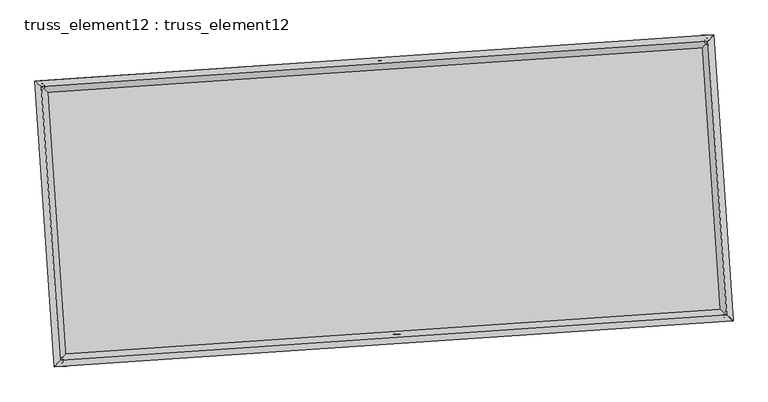
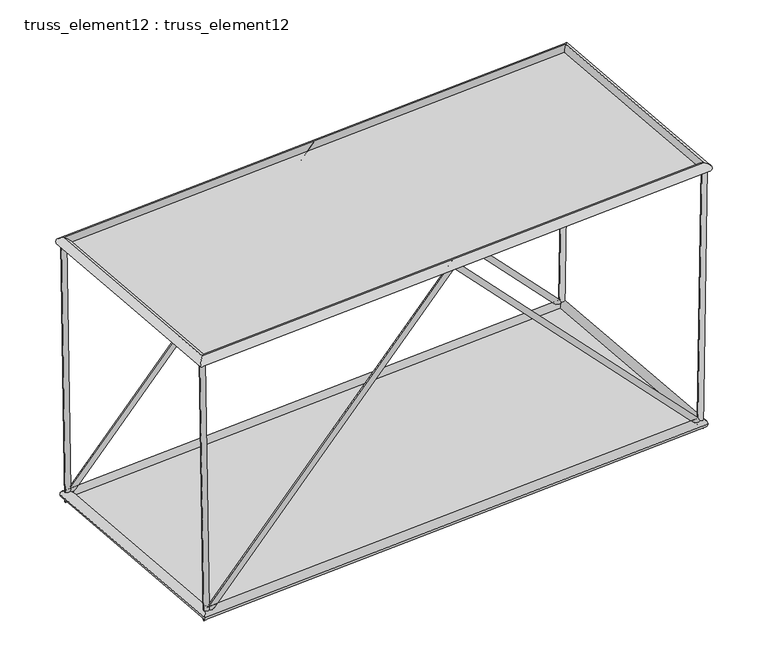
"""IFC4 building model written with IfcOpenShell, lengths in millimetres: plate geometry, truss_element12 : truss_element12."""

from ifc_helpers import new_model, si_unit, frame, origin, origin_with_axes, place, context, project, spatial, polyline, circle_curve, ellipse_curve, outline, extrude, source, transform, mapped, element, save
from ifc_brep_helpers import plane_surface, cylinder_surface, advanced_brep


def truss_element12_truss_element12_4dc9c78d(model_context):
    return source(origin(), model_context, "Body", "SolidModel", [
        advanced_brep(
        [(-3742.1586906, 2270.9588257, 5000.17326), (-3841.2501331, 2257.5984092, 4998.628818), (-3666.8232994, 2276.0956597, 122.2157514), (-3762.1635834, 2262.9910204, -122.2157514), (1064.4043804, 2598.7000901, 5071.5097697), (1064.8423536, 2592.1262061, 4927.2710258), (5794.2950326, 2921.2133537, 122.2062979), (5890.4659444, 2921.1671348, -122.2062979), (5870.9574359, 2926.4406715, 5000.1655764), (5970.9448558, 2926.6546859, 4998.5939366)],
        [
            (0, 1, circle_curve(frame((-3791.7044118, 2264.2786175, 4999.401039), z_axis=(-0.015442194086675787, -0.001052944513496157, 0.9998802077997349), x_axis=(-0.13360442229638714, 0.9910342165763874, -0.0010197635386259769)), 50.0)),
            (1, 0, circle_curve(frame((-3791.7044118, 2264.2786175, 4999.401039), z_axis=(-0.015442194086675787, -0.001052944513496157, 0.9998802077997349), x_axis=(-0.13360442229638714, 0.9910342165763874, -0.0010197635386259769)), 50.0)),
            (0, 2),
            (2, 3, ellipse_curve(frame((-3714.4934414, 2269.54334, 0.0), z_axis=(-0.9286156837382232, -0.06331877347542132, 0.3656003895525282), x_axis=(0.3647534382550642, 0.02487115039698508, 0.9307719136066793)), 131.5917158, 50.0)),
            (3, 1),
            (3, 2, ellipse_curve(frame((-3714.4934414, 2269.54334, 0.0), z_axis=(-0.9286156837382232, -0.06331877347542132, 0.3656003895525282), x_axis=(0.3647534382550642, 0.02487115039698508, 0.9307719136066793)), 131.5917158, 50.0)),
            (2, 4),
            (4, 5, ellipse_curve(frame((1064.623367, 2595.4131481, 4999.3903977), z_axis=(-0.9976833935551671, -0.06802823805689365, 7.107123410103151e-05), x_axis=(-7.090659020090212e-05, -4.834850843570908e-06, -0.9999999974744399)), 72.2764102, 50.0)),
            (5, 3),
            (5, 4, ellipse_curve(frame((1064.623367, 2595.4131481, 4999.3903977), z_axis=(-0.9976833935551671, -0.06802823805689365, 7.107123410103151e-05), x_axis=(-7.090659020090212e-05, -4.834850843570908e-06, -0.9999999974744399)), 72.2764102, 50.0)),
            (4, 6),
            (6, 7, ellipse_curve(frame((5842.3804885, 2921.1902443, 0.0), z_axis=(-0.9286913035150784, -0.06332392970054683, -0.3654073654193971), x_axis=(-0.3645608612823973, -0.024858019305274374, 0.9308477089713738)), 131.5708228, 50.0)),
            (7, 5),
            (7, 6, ellipse_curve(frame((5842.3804885, 2921.1902443, 0.0), z_axis=(-0.9286913035150784, -0.06332392970054683, -0.3654073654193971), x_axis=(-0.3645608612823973, -0.024858019305274374, 0.9308477089713738)), 131.5708228, 50.0)),
            (8, 9, circle_curve(frame((5920.9511458, 2926.5476787, 4999.3797565), z_axis=(0.015714131466516956, 0.0010714868896948503, 0.9998759513000092), x_axis=(-0.0021567180950881, 0.999997135846371, -0.001037721597124432)), 50.0)),
            (9, 8, circle_curve(frame((5920.9511458, 2926.5476787, 4999.3797565), z_axis=(0.015714131466516956, 0.0010714868896948503, 0.9998759513000092), x_axis=(-0.0021567180950881, 0.999997135846371, -0.001037721597124432)), 50.0)),
            (6, 8),
            (9, 7),
        ],
        [
            plane_surface(frame((-3791.7044118, 2314.2785898, 4999.4536925), z_axis=(-0.015442194086678138, -0.0010529445134923887, 0.999880207799735), x_axis=(0.9998807622120698, -1.6261712550758024e-05, 0.015442185524314301))),
            cylinder_surface(frame((-3791.7044118, 2264.2786175, 4999.401039), z_axis=(-0.015442194086675787, -0.001052944513496157, 0.9998802077997349), x_axis=(-0.13360442229638714, 0.9910342165763874, -0.0010197635386259769)), 50.0),
            cylinder_surface(frame((-3714.4934414, 2269.54334, 0.0), z_axis=(-0.6902372461888914, -0.04706465398020624, -0.7220508723900967), x_axis=(-0.020418678997707614, 0.9987519221526339, -0.0455815263501347)), 50.0),
            cylinder_surface(frame((1064.623367, 2595.4131481, 4999.3903977), z_axis=(-0.690134842885581, -0.047057671488226385, 0.7221492049357947), x_axis=(-0.11534864518782999, 0.9922790086207144, -0.045574763894335776)), 50.0),
            plane_surface(frame((5920.9511458, 2876.5477074, 4999.4333375), z_axis=(0.01571413146651804, 0.0010714868896970463, 0.9998759513000093), x_axis=(0.9998765254131398, -1.6839565107673603e-05, -0.01571412244371474))),
            cylinder_surface(frame((5842.3804885, 2921.1902443, 0.0), z_axis=(-0.015714131466516956, -0.0010714868896948503, -0.9998759513000092), x_axis=(-0.0021567180950881, 0.999997135846371, -0.001037721597124432)), 50.0),
        ],
        [
            (0, [[1, 2]]),
            (1, [[-1, 3, 4, 5]]),
            (1, [[-2, -5, 6, -3]]),
            (2, [[-4, 7, 8, 9]]),
            (2, [[-6, -9, 10, -7]]),
            (3, [[-8, 11, 12, 13]]),
            (3, [[-10, -13, 14, -11]]),
            (4, [[15, 16]]),
            (5, [[-12, 17, -16, 18]]),
            (5, [[-14, -18, -15, -17]]),
        ],
    ),
        advanced_brep(
        [(-3470.0457377, -1719.7747586, 5000.17326), (-3569.1371802, -1733.1351751, 4998.628818), (-3394.7103465, -1714.6379246, 122.2157514), (-3490.0506305, -1727.7425639, -122.2157514), (1336.5173333, -1392.0334942, 5071.5097697), (1336.9553065, -1398.6073782, 4927.2710258), (6066.4079855, -1069.5202306, 122.2062979), (6162.5788973, -1069.5664495, -122.2062979), (6143.0703888, -1064.2929128, 5000.1655764), (6243.0578087, -1064.0788984, 4998.5939366)],
        [
            (0, 1, circle_curve(frame((-3519.5914589, -1726.4549668, 4999.401039), z_axis=(-0.01544219408667621, -0.0010529445134962072, 0.9998802077997349), x_axis=(-0.1336044222963871, 0.9910342165763876, -0.0010197635386259834)), 50.0)),
            (1, 0, circle_curve(frame((-3519.5914589, -1726.4549668, 4999.401039), z_axis=(-0.01544219408667621, -0.0010529445134962072, 0.9998802077997349), x_axis=(-0.1336044222963871, 0.9910342165763876, -0.0010197635386259834)), 50.0)),
            (0, 2),
            (2, 3, ellipse_curve(frame((-3442.3804885, -1721.1902443, 0.0), z_axis=(-0.9286156837382233, -0.06331877347542136, 0.3656003895525278), x_axis=(0.3647534382550638, 0.024871150396985044, 0.9307719136066794)), 131.5917158, 50.0)),
            (3, 1),
            (3, 2, ellipse_curve(frame((-3442.3804885, -1721.1902443, 0.0), z_axis=(-0.9286156837382233, -0.06331877347542136, 0.3656003895525278), x_axis=(0.3647534382550638, 0.024871150396985044, 0.9307719136066794)), 131.5917158, 50.0)),
            (2, 4),
            (4, 5, ellipse_curve(frame((1336.7363199, -1395.3204362, 4999.3903977), z_axis=(-0.9976833935551669, -0.0680282380568936, 7.107123409958704e-05), x_axis=(-7.090659019997968e-05, -4.8348508435516935e-06, -0.9999999974744398)), 72.2764102, 50.0)),
            (5, 3),
            (5, 4, ellipse_curve(frame((1336.7363199, -1395.3204362, 4999.3903977), z_axis=(-0.9976833935551669, -0.0680282380568936, 7.107123409958704e-05), x_axis=(-7.090659019997968e-05, -4.8348508435516935e-06, -0.9999999974744398)), 72.2764102, 50.0)),
            (4, 6),
            (6, 7, ellipse_curve(frame((6114.4934414, -1069.54334, 0.0), z_axis=(-0.9286913035150779, -0.06332392970054657, -0.36540736541939867), x_axis=(-0.3645608612823989, -0.024858019305274558, 0.9308477089713731)), 131.5708228, 50.0)),
            (7, 5),
            (7, 6, ellipse_curve(frame((6114.4934414, -1069.54334, 0.0), z_axis=(-0.9286913035150779, -0.06332392970054657, -0.36540736541939867), x_axis=(-0.3645608612823989, -0.024858019305274558, 0.9308477089713731)), 131.5708228, 50.0)),
            (8, 9, circle_curve(frame((6193.0640987, -1064.1859056, 4999.3797565), z_axis=(0.015714131466516297, 0.001071486889694649, 0.9998759513000093), x_axis=(-0.002156718095087732, 0.999997135846371, -0.0010377215971242378)), 50.0)),
            (9, 8, circle_curve(frame((6193.0640987, -1064.1859056, 4999.3797565), z_axis=(0.015714131466516297, 0.001071486889694649, 0.9998759513000093), x_axis=(-0.002156718095087732, 0.999997135846371, -0.0010377215971242378)), 50.0)),
            (6, 8),
            (9, 7),
        ],
        [
            plane_surface(frame((-3519.5914589, -1676.4549945, 4999.4536925), z_axis=(-0.015442194086678138, -0.0010529445134923802, 0.999880207799735), x_axis=(0.9998807622120698, -1.6261712550758024e-05, 0.015442185524314301))),
            cylinder_surface(frame((-3519.5914589, -1726.4549668, 4999.401039), z_axis=(-0.015442194086676214, -0.0010529445134962075, 0.9998802077997351), x_axis=(-0.1336044222963871, 0.9910342165763876, -0.0010197635386259834)), 50.0),
            cylinder_surface(frame((-3442.3804885, -1721.1902443, 0.0), z_axis=(-0.690237246188891, -0.04706465398020623, -0.722050872390097), x_axis=(-0.020418678997707614, 0.9987519221526338, -0.04558152635013466)), 50.0),
            cylinder_surface(frame((1336.7363199, -1395.3204362, 4999.3903977), z_axis=(-0.6901348428855829, -0.0470576714882265, 0.7221492049357932), x_axis=(-0.11534864518782982, 0.9922790086207144, -0.04557476389433585)), 50.0),
            plane_surface(frame((6193.0640987, -1114.1858769, 4999.4333375), z_axis=(0.01571413146651804, 0.001071486889697036, 0.9998759513000093), x_axis=(0.9998765254131398, -1.6839565107673603e-05, -0.01571412244371474))),
            cylinder_surface(frame((6114.4934414, -1069.54334, 0.0), z_axis=(-0.015714131466516297, -0.001071486889694649, -0.9998759513000093), x_axis=(-0.002156718095087732, 0.999997135846371, -0.0010377215971242378)), 50.0),
        ],
        [
            (0, [[1, 2]]),
            (1, [[-1, 3, 4, 5]]),
            (1, [[-2, -5, 6, -3]]),
            (2, [[-4, 7, 8, 9]]),
            (2, [[-6, -9, 10, -7]]),
            (3, [[-8, 11, 12, 13]]),
            (3, [[-10, -13, 14, -11]]),
            (4, [[15, 16]]),
            (5, [[-12, 17, -16, 18]]),
            (5, [[-14, -18, -15, -17]]),
        ],
    ),
        advanced_brep(
        [(-3519.5970265, -1726.4611376, 4909.4010392), (-3519.5858913, -1726.448796, 5089.4010388), (-3791.6980582, 2264.2732596, 5089.4010388), (-3791.7107655, 2264.2839754, 4909.4010392), (5920.9459708, 2926.5415347, 5089.3797563), (5920.9563208, 2926.5538227, 4909.3797567), (6193.0581377, -1064.1805209, 5089.3797563), (6193.0700598, -1064.1912903, 4909.3797567)],
        [
            (0, 1, ellipse_curve(frame((-3519.5914589, -1726.4549668, 4999.401039), z_axis=(-0.7535719234037699, 0.6573654662781984, 1.545832286464647e-06), x_axis=(-0.6573654662763975, -0.7535719234053407, 1.5458322803391796e-06)), 127.2792206, 90.0)),
            (1, 2),
            (2, 3, ellipse_curve(frame((-3791.7044118, 2264.2786175, 4999.401039), z_axis=(-0.6573654662763976, -0.7535719234053407, 1.5458322815977818e-06), x_axis=(0.7535719234037699, -0.6573654662781983, -1.5458322877232492e-06)), 127.2792206, 90.0)),
            (3, 0),
            (1, 0, ellipse_curve(frame((-3519.5914589, -1726.4549668, 4999.401039), z_axis=(-0.7535719234037699, 0.6573654662781984, 1.545832286464647e-06), x_axis=(-0.6573654662763975, -0.7535719234053407, 1.5458322803391796e-06)), 127.2792206, 90.0)),
            (3, 2, ellipse_curve(frame((-3791.7044118, 2264.2786175, 4999.401039), z_axis=(-0.6573654662763976, -0.7535719234053407, 1.5458322815977818e-06), x_axis=(0.7535719234037699, -0.6573654662781983, -1.5458322877232492e-06)), 127.2792206, 90.0)),
            (2, 4),
            (4, 5, ellipse_curve(frame((5920.9511458, 2926.5476787, 4999.3797565), z_axis=(-0.7535719234037713, 0.6573654662781966, 1.5458322846605871e-06), x_axis=(-0.6573654662763959, -0.7535719234053422, 1.545832284660444e-06)), 127.2792206, 90.0)),
            (5, 3),
            (5, 4, ellipse_curve(frame((5920.9511458, 2926.5476787, 4999.3797565), z_axis=(-0.7535719234037713, 0.6573654662781966, 1.5458322846605871e-06), x_axis=(-0.6573654662763959, -0.7535719234053422, 1.545832284660444e-06)), 127.2792206, 90.0)),
            (4, 6),
            (6, 7, ellipse_curve(frame((6193.0640987, -1064.1859056, 4999.3797565), z_axis=(0.6573654662763961, 0.7535719234053421, -1.5458322834018422e-06), x_axis=(-0.7535719234037712, 0.6573654662781966, 1.5458322834019847e-06)), 127.2792206, 90.0)),
            (7, 5),
            (7, 6, ellipse_curve(frame((6193.0640987, -1064.1859056, 4999.3797565), z_axis=(0.6573654662763961, 0.7535719234053421, -1.5458322834018422e-06), x_axis=(-0.7535719234037712, 0.6573654662781966, 1.5458322834019847e-06)), 127.2792206, 90.0)),
            (6, 1),
            (0, 7),
        ],
        [
            cylinder_surface(frame((-3519.5914589, -1726.4549668, 4999.401039), z_axis=(0.06802823822869561, -0.997683396074877, 0.0), x_axis=(-0.9976833938766201, -0.06802823807880483, 6.638314775147211e-05)), 90.0),
            cylinder_surface(frame((-3791.7044118, 2264.2786175, 4999.401039), z_axis=(-0.9976833960724927, -0.06802823822853761, 2.1861369821210883e-06), x_axis=(-0.06802823794850094, 0.9976833940285695, 6.419701077818742e-05)), 90.0),
            cylinder_surface(frame((5920.9511458, 2926.5476787, 4999.3797565), z_axis=(-0.06802823822869979, 0.9976833960748769, 0.0), x_axis=(0.9976833941566566, 0.06802823809790365, 6.201087380057128e-05)), 90.0),
            cylinder_surface(frame((6193.0640987, -1064.1859056, 4999.3797565), z_axis=(0.9976833960724927, 0.06802823822853742, -2.186136980341156e-06), x_axis=(0.06802823822853742, -0.9976833940094749, 6.419701077640772e-05)), 90.0),
        ],
        [
            (0, [[1, 2, 3, 4]]),
            (0, [[5, -4, 6, -2]]),
            (1, [[-3, 7, 8, 9]]),
            (1, [[-6, -9, 10, -7]]),
            (2, [[-8, 11, 12, 13]]),
            (2, [[-10, -13, 14, -11]]),
            (3, [[-12, 15, -1, 16]]),
            (3, [[-14, -16, -5, -15]]),
        ],
    ),
        advanced_brep(
        [(-3358.7115243, -1625.2761972, 0.0), (-3526.0494527, -1817.1042913, 0.0), (-3810.4074885, 2353.2123043, 0.0), (-3618.5793943, 2185.8743758, 0.0), (5926.0494527, 3017.1042913, 0.0), (5758.7115243, 2825.2761972, 0.0), (6210.4074885, -1153.2123043, 0.0), (6018.5793943, -985.8743758, 0.0)],
        [
            (0, 1, ellipse_curve(frame((-3442.3804885, -1721.1902443, 0.0), z_axis=(-0.7535719234054578, 0.6573654662780809, 0.0), x_axis=(-0.6573654662780807, -0.7535719234054579, 0.0)), 127.2792206, 90.0)),
            (1, 2),
            (2, 3, ellipse_curve(frame((-3714.4934414, 2269.54334, 0.0), z_axis=(-0.6573654662780809, -0.7535719234054579, 0.0), x_axis=(0.7535719234054578, -0.6573654662780809, 0.0)), 127.2792206, 90.0)),
            (3, 0),
            (1, 0, ellipse_curve(frame((-3442.3804885, -1721.1902443, 0.0), z_axis=(-0.7535719234054578, 0.6573654662780809, 0.0), x_axis=(-0.6573654662780807, -0.7535719234054579, 0.0)), 127.2792206, 90.0)),
            (3, 2, ellipse_curve(frame((-3714.4934414, 2269.54334, 0.0), z_axis=(-0.6573654662780809, -0.7535719234054579, 0.0), x_axis=(0.7535719234054578, -0.6573654662780809, 0.0)), 127.2792206, 90.0)),
            (2, 4),
            (4, 5, ellipse_curve(frame((5842.3804885, 2921.1902443, 0.0), z_axis=(-0.7535719234054592, 0.6573654662780795, 0.0), x_axis=(-0.6573654662780793, -0.7535719234054592, 0.0)), 127.2792206, 90.0)),
            (5, 3),
            (5, 4, ellipse_curve(frame((5842.3804885, 2921.1902443, 0.0), z_axis=(-0.7535719234054592, 0.6573654662780795, 0.0), x_axis=(-0.6573654662780793, -0.7535719234054592, 0.0)), 127.2792206, 90.0)),
            (4, 6),
            (6, 7, ellipse_curve(frame((6114.4934414, -1069.54334, 0.0), z_axis=(0.6573654662780795, 0.7535719234054591, 0.0), x_axis=(-0.7535719234054591, 0.6573654662780795, 0.0)), 127.2792206, 90.0)),
            (7, 5),
            (7, 6, ellipse_curve(frame((6114.4934414, -1069.54334, 0.0), z_axis=(0.6573654662780795, 0.7535719234054591, 0.0), x_axis=(-0.7535719234054591, 0.6573654662780795, 0.0)), 127.2792206, 90.0)),
            (6, 1),
            (0, 7),
        ],
        [
            cylinder_surface(frame((-3442.3804885, -1721.1902443, 0.0), z_axis=(0.06802823822869894, -0.9976833960748769, 0.0), x_axis=(-0.9976833960748769, -0.06802823822869894, 0.0)), 90.0),
            cylinder_surface(frame((-3714.4934414, 2269.54334, 0.0), z_axis=(-0.9976833960748765, -0.06802823822870331, 0.0), x_axis=(-0.06802823822870331, 0.9976833960748765, 0.0)), 90.0),
            cylinder_surface(frame((5842.3804885, 2921.1902443, 0.0), z_axis=(-0.06802823822870283, 0.9976833960748765, 0.0), x_axis=(0.9976833960748765, 0.06802823822870283, 0.0)), 90.0),
            cylinder_surface(frame((6114.4934414, -1069.54334, 0.0), z_axis=(0.9976833960748765, 0.06802823822870317, 0.0), x_axis=(0.06802823822870317, -0.9976833960748765, 0.0)), 90.0),
        ],
        [
            (0, [[1, 2, 3, 4]]),
            (0, [[5, -4, 6, -2]]),
            (1, [[-3, 7, 8, 9]]),
            (1, [[-6, -9, 10, -7]]),
            (2, [[-8, 11, 12, 13]]),
            (2, [[-10, -13, 14, -11]]),
            (3, [[-12, 15, -1, 16]]),
            (3, [[-14, -16, -5, -15]]),
        ],
    ),
        extrude(outline(polyline([(-3442.3804885, -1721.1902443), (-3714.4934414, 2269.54334), (5842.3804885, 2921.1902443), (6114.4934414, -1069.54334), (-3442.3804885, -1721.1902443)])), origin_with_axes(), (0.0, 0.0, 1.0), 20.0),
        extrude(outline(polyline([(-1999.9999999, 4867.6040895), (2000.0000001, 4867.6040895), (2000.0, -4867.6040896), (-2000.0, -4867.6040896), (-1999.9999999, 4867.6040895)])), frame((1200.6798434, 600.0463559, 4999.3903977), z_axis=(2.1810725689020035e-06, 1.4871904309886001e-07, 0.9999999999976105), x_axis=(-0.0680282382286986, 0.9976833960748768, 0.0)), (0.0, 0.0, 1.0), 20.0),
    ])


if __name__ == "__main__":
    model = new_model("IFC4")
    model_context = context("Model", 3, world=origin())
    ifc_project = project(units=[si_unit("LENGTHUNIT", "METRE", prefix="MILLI")], contexts=[model_context])
    site = spatial("IfcSite", under=ifc_project)
    building = spatial("IfcBuilding", under=site)
    placement = place(None, origin())
    truss_element12_truss_element12_shape = truss_element12_truss_element12_4dc9c78d(model_context)
    element("IfcPlate", 1, ObjectType="truss_element12 : truss_element12", at=placement, inside=building, context=model_context, shape_type="MappedRepresentation", body=[
        mapped(truss_element12_truss_element12_shape, transform((0.0, 0.0, 0.0), x_axis=(1.0, 0.0, 0.0), y_axis=(0.0, 1.0, 0.0), z_axis=(0.0, 0.0, 1.0))),
    ])
    save(model, "model.ifc")

# Revit data of these elements
# Type "truss_element12 : truss_element12"
#   steellbar1 = 90 mm
#   steelbar2 = 50 mm
#   offset1 = 5000 mm
#   M = Default Roof
# Element 1 (IfcPlate, "truss_element12 : truss_element12")
#   Materials on its faces: "Default Roof"
# Materials
#   "Default Roof": class "Miscellaneous", colour RGB 0 127 0, transparency 0, Comments = "Rendering appearance not upgraded Rendering appearance not upgraded ", Cost = 0
